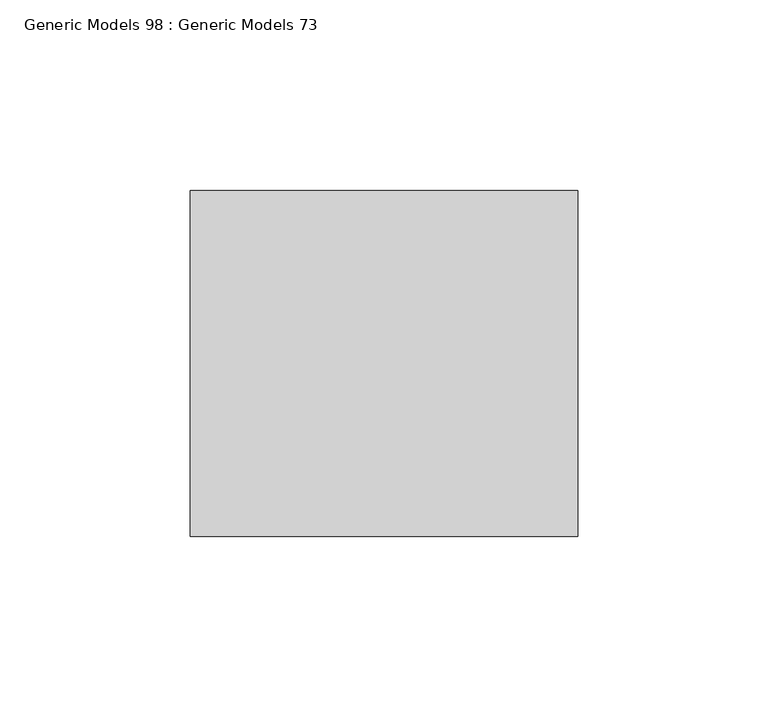
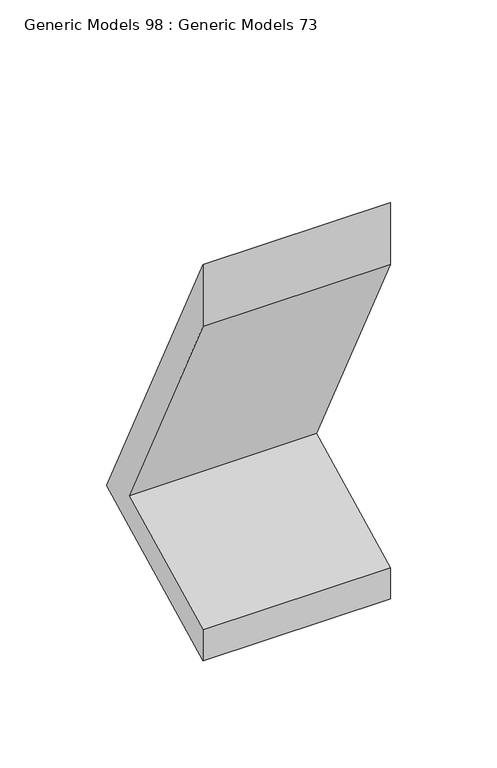
"""IFC4 building model written with IfcOpenShell, lengths in millimetres: proxy geometry, Generic Models 98 : Generic Models 73."""

from ifc_helpers import new_model, si_unit, frame, origin, place, context, project, spatial, polyline, outline, extrude, source, transform, mapped, element, save


def generic_models_98_generic_models_73_d1751a9c(model_context):
    return source(origin(), model_context, "Body", "SweptSolid", [
        extrude(outline(polyline([(30949.3519638, 269191.7744013), (30858.4781612, 269146.3375), (30858.4781612, 269164.0862896), (30928.0534163, 269198.8739171), (30858.4781612, 269338.0244274), (30858.4781612, 269373.5220065), (30949.3519638, 269191.7744013)])), frame((31924.6096032, 0.0, 0.0), z_axis=(1.0, 0.0, 0.0), x_axis=(0.0, 1.0, 0.0)), (0.0, 0.0, 1.0), 101.6),
    ])


if __name__ == "__main__":
    model = new_model("IFC4")
    model_context = context("Model", 3, world=origin())
    ifc_project = project(units=[si_unit("LENGTHUNIT", "METRE", prefix="MILLI")], contexts=[model_context])
    site = spatial("IfcSite", under=ifc_project)
    building = spatial("IfcBuilding", under=site)
    placement = place(None, origin())
    generic_models_98_generic_models_73_shape = generic_models_98_generic_models_73_d1751a9c(model_context)
    element("IfcBuildingElementProxy", 1, Name="Generic Models 98 : Generic Models 73", ObjectType="Generic Models 98 : Generic Models 73", at=placement, inside=building, context=model_context, shape_type="MappedRepresentation", body=[
        mapped(generic_models_98_generic_models_73_shape, transform((0.0, 0.0, 0.0), x_axis=(1.0, 0.0, 0.0), y_axis=(0.0, 1.0, 0.0), z_axis=(0.0, 0.0, 1.0))),
    ])
    save(model, "model.ifc")

# Revit data of these elements
# Element 1 (IfcBuildingElementProxy, "Generic Models 98 : Generic Models 73")
#   Materials on its faces: "L8 x 4 x 5/8 x 0'-4\" METAL ANGLE"
# Materials
#   "L8 x 4 x 5/8 x 0'-4\" METAL ANGLE": class "Metal", colour RGB 199 199 199, transparency 0, Description = "Carbon steel", Cost = 0
